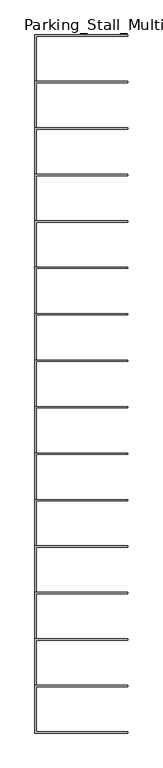
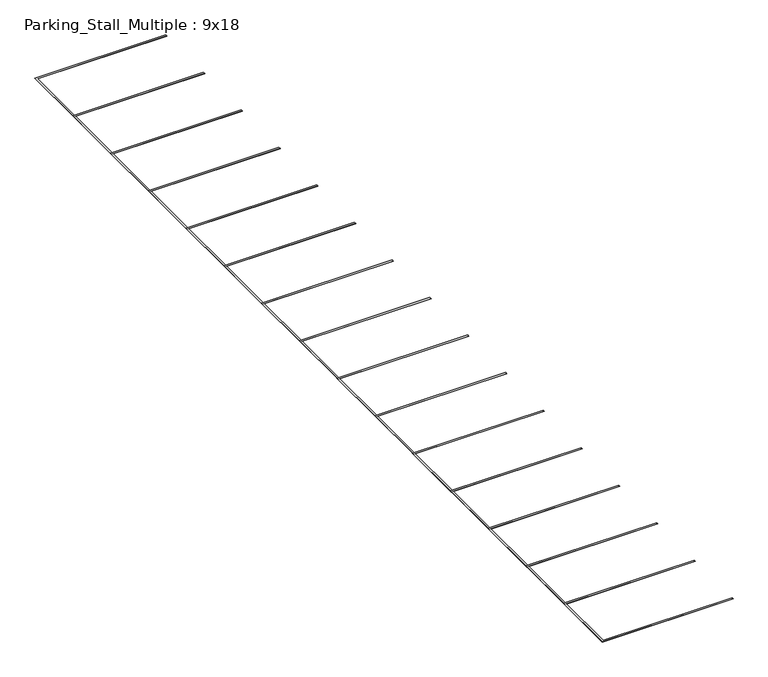
"""IFC4 building model written with IfcOpenShell, lengths in millimetres: proxy geometry, Parking_Stall_Multiple : 9x18."""

import ifcopenshell
import ifcopenshell.guid

model = None  # the IFC model being written
_history = None  # IfcOwnerHistory: only IFC2X3 demands one
_inside = {}  # id of a spatial element -> (the spatial element, [elements in it])
_under = {}  # id of a project, library or spatial element -> (it, [spatial elements below it])
_declared = {}  # id of a project -> (the project, [libraries it declares])
_typed = {}  # id of a type object -> (the type object, [elements of that type])
_made_of = {}  # id of a material, layer set ... -> (it, [elements and type objects made of it])


def new_model(schema):
    """Start an empty IFC model of exactly this schema.

    Asked for "IFC4X3", IfcOpenShell would pick the latest addendum, in which some entities
    have other attributes; the version numbers below select the first issue.
    IFC2X3 requires an IfcOwnerHistory on every rooted entity: one is made here for all.
    """
    global model, _history
    if schema == "IFC4X3":
        model = ifcopenshell.file(schema_version=(4, 3, 0, 0))
    else:
        model = ifcopenshell.file(schema=schema)
    _inside.clear()
    _under.clear()
    _declared.clear()
    _typed.clear()
    _made_of.clear()
    _history = None
    if model.schema == "IFC2X3":
        org = make("IfcOrganization", Name="unknown")
        user = make(
            "IfcPersonAndOrganization",
            ThePerson=make("IfcPerson", FamilyName="unknown"),
            TheOrganization=org,
        )
        app = make(
            "IfcApplication",
            ApplicationDeveloper=org,
            Version="unknown",
            ApplicationFullName="unknown",
            ApplicationIdentifier="unknown",
        )
        _history = make(
            "IfcOwnerHistory",
            OwningUser=user,
            OwningApplication=app,
            ChangeAction="ADDED",
            CreationDate=0,
        )
    return model


def make(cls, **values):
    """One entity of the class cls with the attributes given. An attribute that is None is left unset."""
    return model.create_entity(
        cls, **{name: value for name, value in values.items() if value is not None}
    )


def rooted(cls, **values):
    """An entity with a GlobalId (a new one), such as an element, a storey or a relation."""
    return make(cls, GlobalId=ifcopenshell.guid.new(), OwnerHistory=_history, **values)


def si_unit(unit_type, name, prefix=None):
    """IfcSIUnit, for example si_unit("LENGTHUNIT", "METRE", prefix="MILLI")."""
    return make("IfcSIUnit", UnitType=unit_type, Prefix=prefix, Name=name)


def assignment(units):
    """IfcUnitAssignment: the units of a project."""
    return None if units is None else make("IfcUnitAssignment", Units=units)


def point(xyz):
    """IfcCartesianPoint."""
    return None if xyz is None else make("IfcCartesianPoint", Coordinates=xyz)


def direction(xyz):
    """IfcDirection."""
    return None if xyz is None else make("IfcDirection", DirectionRatios=xyz)


def frame(location, z_axis=None, x_axis=None):
    """IfcAxis2Placement3D, a coordinate frame: its origin and axes. An axis left out is left unset."""
    return make(
        "IfcAxis2Placement3D",
        Location=point(location),
        Axis=direction(z_axis),
        RefDirection=direction(x_axis),
    )


def origin():
    """The frame at (0, 0, 0) with its axes left unset."""
    return frame((0.0, 0.0, 0.0))


def origin_with_axes():
    """The frame at (0, 0, 0) with the z axis (0, 0, 1) and the x axis (1, 0, 0) written out."""
    return frame((0.0, 0.0, 0.0), z_axis=(0.0, 0.0, 1.0), x_axis=(1.0, 0.0, 0.0))


def place(relative_to, where):
    """IfcLocalPlacement: puts the frame where relative to a parent placement (None: the world)."""
    return make(
        "IfcLocalPlacement", PlacementRelTo=relative_to, RelativePlacement=where
    )


def context(
    kind, dimensions, precision=None, world=None, true_north=None, identifier=None
):
    """IfcGeometricRepresentationContext, for example the 3D "Model" context."""
    return make(
        "IfcGeometricRepresentationContext",
        ContextIdentifier=identifier,
        ContextType=kind,
        CoordinateSpaceDimension=dimensions,
        Precision=precision,
        WorldCoordinateSystem=world,
        TrueNorth=true_north,
    )


def project(units=None, contexts=None):
    """IfcProject with its units and contexts."""
    return rooted(
        "IfcProject",
        Name="project",
        RepresentationContexts=contexts,
        UnitsInContext=assignment(units),
    )


def spatial(cls, under=None, at=None, **own):
    """A site, building, storey or space (cls), placed at a placement, below another one or the project."""
    s = rooted(cls, ObjectPlacement=at, **own)
    if under is not None:
        _under.setdefault(under.id(), (under, []))[1].append(s)
    return s


def polyline(points):
    """IfcPolyline through the points."""
    return make("IfcPolyline", Points=[point(p) for p in points])


def outline(outer, holes=None, kind="AREA"):
    """IfcArbitraryClosedProfileDef: a profile drawn as a closed curve; with holes, ...WithVoids."""
    if holes is None:
        return make("IfcArbitraryClosedProfileDef", ProfileType=kind, OuterCurve=outer)
    return make(
        "IfcArbitraryProfileDefWithVoids",
        ProfileType=kind,
        OuterCurve=outer,
        InnerCurves=holes,
    )


def extrude(swept, where, along, depth):
    """IfcExtrudedAreaSolid: the profile swept, set in the frame where, extruded along a direction by depth."""
    return make(
        "IfcExtrudedAreaSolid",
        SweptArea=swept,
        Position=where,
        ExtrudedDirection=direction(along),
        Depth=depth,
    )


def shape(context_of_items, identifier, shape_type, items):
    """IfcShapeRepresentation: the items that make up one representation, for example the "Body"."""
    return make(
        "IfcShapeRepresentation",
        ContextOfItems=context_of_items,
        RepresentationIdentifier=identifier,
        RepresentationType=shape_type,
        Items=items,
    )


def source(mapping_origin, context_of_items, identifier, shape_type, items):
    """IfcRepresentationMap: a shape defined once, which mapped items show again and again."""
    return make(
        "IfcRepresentationMap",
        MappingOrigin=mapping_origin,
        MappedRepresentation=shape(context_of_items, identifier, shape_type, items),
    )


def transform(
    local_origin,
    x_axis=None,
    y_axis=None,
    z_axis=None,
    scale=None,
    scale2=None,
    scale3=None,
    uniform=True,
):
    """IfcCartesianTransformationOperator3D, or its non-uniform kind. x_axis, y_axis, z_axis: its Axis1, 2, 3."""
    if uniform:
        return make(
            "IfcCartesianTransformationOperator3D",
            Axis1=direction(x_axis),
            Axis2=direction(y_axis),
            LocalOrigin=point(local_origin),
            Scale=scale,
            Axis3=direction(z_axis),
        )
    return make(
        "IfcCartesianTransformationOperator3DnonUniform",
        Axis1=direction(x_axis),
        Axis2=direction(y_axis),
        LocalOrigin=point(local_origin),
        Scale=scale,
        Axis3=direction(z_axis),
        Scale2=scale2,
        Scale3=scale3,
    )


def mapped(mapping_source, mapping_target):
    """IfcMappedItem: shows the shape of a source again, moved by a transform."""
    return make(
        "IfcMappedItem", MappingSource=mapping_source, MappingTarget=mapping_target
    )


def made_of(thing, what):
    """Note that an element or type object is made of a material, layer set ...; save() writes the relation."""
    if what is not None:
        _made_of.setdefault(what.id(), (what, []))[1].append(thing)
    return thing


def element(
    cls,
    number,
    at=None,
    inside=None,
    cuts=None,
    type_object=None,
    material=None,
    context=None,
    identifier="Body",
    shape_type=None,
    held_by="IfcProductDefinitionShape",
    body=None,
    shapes=None,
    **own,
):
    """One element of the class cls, such as IfcWall. Its Tag is "e" and its number.

    at: its placement. inside: the storey or other place that contains it. cuts: it is an
    opening in that element (IfcRelVoidsElement). A single representation is given by context,
    identifier, shape_type and body (its items); several are given by shapes. held_by: the class
    of the entity that holds the representations. save() writes the other relations.
    """
    e = rooted(cls, Tag="e%d" % number, ObjectPlacement=at, **own)
    if body is not None:
        shapes = [shape(context, identifier, shape_type, body)]
    if shapes is not None:
        e.Representation = make(held_by, Representations=shapes)
    if inside is not None:
        _inside.setdefault(inside.id(), (inside, []))[1].append(e)
    if cuts is not None:
        rooted(
            "IfcRelVoidsElement", RelatingBuildingElement=cuts, RelatedOpeningElement=e
        )
    if type_object is not None:
        _typed.setdefault(type_object.id(), (type_object, []))[1].append(e)
    return made_of(e, material)


def aggregate(whole, parts):
    """IfcRelAggregates: a whole, such as a stair, and the parts it consists of."""
    return rooted("IfcRelAggregates", RelatingObject=whole, RelatedObjects=parts)


def save(model, path):
    """Write the relations noted so far, then the file.

    IfcRelAggregates (storeys below a building ...), IfcRelContainedInSpatialStructure (elements
    in a storey), IfcRelDefinesByType, IfcRelAssociatesMaterial and IfcRelDeclares: one each for
    every whole, place, type object, material and project.
    """
    for whole, parts in _under.values():
        aggregate(whole, parts)
    for where, things in _inside.values():
        rooted(
            "IfcRelContainedInSpatialStructure",
            RelatedElements=things,
            RelatingStructure=where,
        )
    for kind, things in _typed.values():
        rooted("IfcRelDefinesByType", RelatedObjects=things, RelatingType=kind)
    for what, things in _made_of.values():
        rooted("IfcRelAssociatesMaterial", RelatedObjects=things, RelatingMaterial=what)
    for by, libraries in _declared.values():
        rooted("IfcRelDeclares", RelatingContext=by, RelatedDefinitions=libraries)
    model.write(path)


def parking_stall_multiple_9x18_58801655(model_context):
    return source(origin(), model_context, "Body", "SweptSolid", [
        extrude(outline(polyline([(5486.4, -38404.8), (5486.4, -38481.0), (76.2, -38481.0), (76.2, -41148.0), (5486.4, -41148.0), (5486.4, -41224.2), (0.0, -41224.2), (0.0, -38404.8), (5486.4, -38404.8)])), origin_with_axes(), (0.0, 0.0, 1.0), 6.35),
        extrude(outline(polyline([(5486.4, -35661.6), (5486.4, -35737.8), (76.2, -35737.8), (76.2, -38404.8), (5486.4, -38404.8), (5486.4, -38481.0), (0.0, -38481.0), (0.0, -35661.6), (5486.4, -35661.6)])), origin_with_axes(), (0.0, 0.0, 1.0), 6.35),
        extrude(outline(polyline([(5486.4, -32918.4), (5486.4, -32994.6), (76.2, -32994.6), (76.2, -35661.6), (5486.4, -35661.6), (5486.4, -35737.8), (0.0, -35737.8), (0.0, -32918.4), (5486.4, -32918.4)])), origin_with_axes(), (0.0, 0.0, 1.0), 6.35),
        extrude(outline(polyline([(5486.4, -30175.2), (5486.4, -30251.4), (76.2, -30251.4), (76.2, -32918.4), (5486.4, -32918.4), (5486.4, -32994.6), (0.0, -32994.6), (0.0, -30175.2), (5486.4, -30175.2)])), origin_with_axes(), (0.0, 0.0, 1.0), 6.35),
        extrude(outline(polyline([(5486.4, -27432.0), (5486.4, -27508.2), (76.2, -27508.2), (76.2, -30175.2), (5486.4, -30175.2), (5486.4, -30251.4), (0.0, -30251.4), (0.0, -27432.0), (5486.4, -27432.0)])), origin_with_axes(), (0.0, 0.0, 1.0), 6.35),
        extrude(outline(polyline([(5486.4, -24688.8), (5486.4, -24765.0), (76.2, -24765.0), (76.2, -27432.0), (5486.4, -27432.0), (5486.4, -27508.2), (0.0, -27508.2), (0.0, -24688.8), (5486.4, -24688.8)])), origin_with_axes(), (0.0, 0.0, 1.0), 6.35),
        extrude(outline(polyline([(5486.4, -21945.6), (5486.4, -22021.8), (76.2, -22021.8), (76.2, -24688.8), (5486.4, -24688.8), (5486.4, -24765.0), (0.0, -24765.0), (0.0, -21945.6), (5486.4, -21945.6)])), origin_with_axes(), (0.0, 0.0, 1.0), 6.35),
        extrude(outline(polyline([(5486.4, -19202.4), (5486.4, -19278.6), (76.2, -19278.6), (76.2, -21945.6), (5486.4, -21945.6), (5486.4, -22021.8), (0.0, -22021.8), (0.0, -19202.4), (5486.4, -19202.4)])), origin_with_axes(), (0.0, 0.0, 1.0), 6.35),
        extrude(outline(polyline([(5486.4, -16459.2), (5486.4, -16535.4), (76.2, -16535.4), (76.2, -19202.4), (5486.4, -19202.4), (5486.4, -19278.6), (0.0, -19278.6), (0.0, -16459.2), (5486.4, -16459.2)])), origin_with_axes(), (0.0, 0.0, 1.0), 6.35),
        extrude(outline(polyline([(5486.4, -13716.0), (5486.4, -13792.2), (76.2, -13792.2), (76.2, -16459.2), (5486.4, -16459.2), (5486.4, -16535.4), (0.0, -16535.4), (0.0, -13716.0), (5486.4, -13716.0)])), origin_with_axes(), (0.0, 0.0, 1.0), 6.35),
        extrude(outline(polyline([(5486.4, -10972.8), (5486.4, -11049.0), (76.2, -11049.0), (76.2, -13716.0), (5486.4, -13716.0), (5486.4, -13792.2), (0.0, -13792.2), (0.0, -10972.8), (5486.4, -10972.8)])), origin_with_axes(), (0.0, 0.0, 1.0), 6.35),
        extrude(outline(polyline([(5486.4, -8229.6), (5486.4, -8305.8), (76.2, -8305.8), (76.2, -10972.8), (5486.4, -10972.8), (5486.4, -11049.0), (0.0, -11049.0), (0.0, -8229.6), (5486.4, -8229.6)])), origin_with_axes(), (0.0, 0.0, 1.0), 6.35),
        extrude(outline(polyline([(5486.4, -5486.4), (5486.4, -5562.6), (76.2, -5562.6), (76.2, -8229.6), (5486.4, -8229.6), (5486.4, -8305.8), (0.0, -8305.8), (0.0, -5486.4), (5486.4, -5486.4)])), origin_with_axes(), (0.0, 0.0, 1.0), 6.35),
        extrude(outline(polyline([(5486.4, -2743.2), (5486.4, -2819.4), (76.2, -2819.4), (76.2, -5486.4), (5486.4, -5486.4), (5486.4, -5562.6), (0.0, -5562.6), (0.0, -2743.2), (5486.4, -2743.2)])), origin_with_axes(), (0.0, 0.0, 1.0), 6.35),
        extrude(outline(polyline([(5486.4, 0.0), (5486.4, -76.2), (76.2, -76.2), (76.2, -2743.2), (5486.4, -2743.2), (5486.4, -2819.4), (0.0, -2819.4), (0.0, 0.0), (5486.4, 0.0)])), origin_with_axes(), (0.0, 0.0, 1.0), 6.35),
    ])


if __name__ == "__main__":
    model = new_model("IFC4")
    model_context = context("Model", 3, world=origin())
    ifc_project = project(units=[si_unit("LENGTHUNIT", "METRE", prefix="MILLI")], contexts=[model_context])
    site = spatial("IfcSite", under=ifc_project)
    building = spatial("IfcBuilding", under=site)
    placement = place(None, origin())
    parking_stall_multiple_9x18_shape = parking_stall_multiple_9x18_58801655(model_context)
    element("IfcBuildingElementProxy", 1, Name="Parking_Stall_Multiple : 9x18", ObjectType="Parking_Stall_Multiple : 9x18", at=placement, inside=building, context=model_context, shape_type="MappedRepresentation", body=[
        mapped(parking_stall_multiple_9x18_shape, transform((0.0, 0.0, 0.0), x_axis=(1.0, 0.0, 0.0), y_axis=(0.0, 1.0, 0.0), z_axis=(0.0, 0.0, 1.0))),
    ])
    save(model, "model.ifc")

# Revit data of these elements
# Type "Parking_Stall_Multiple : 9x18"
#   Parking_Width_M = 9' - 0"
#   Parking_Run_Length [instance default] = 65' - 0"
#   Parking_Line_Width = 0' - 3"
#   Parking_Length_M = 18' - 0"
#   Single_Parking_Visibility [instance default] = no
#   Parking_ADA_Symbol = no
#   ParkingUnitsArray [instance default] = 7
#   ParkingUnits [instance default] = 7
#   Multiple_Parking_Visibility [instance default] = yes
#   Parking_Line_Material = none
# Element 1 (IfcBuildingElementProxy, "Parking_Stall_Multiple : 9x18")
#   Parking_Run_Length = 135' - 8.5365"
#   ParkingUnitsArray = 15
#   ParkingUnits = 15
